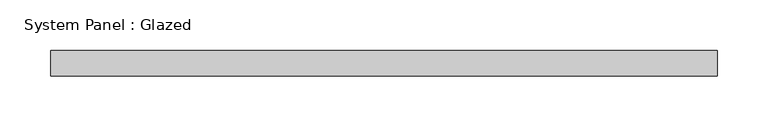
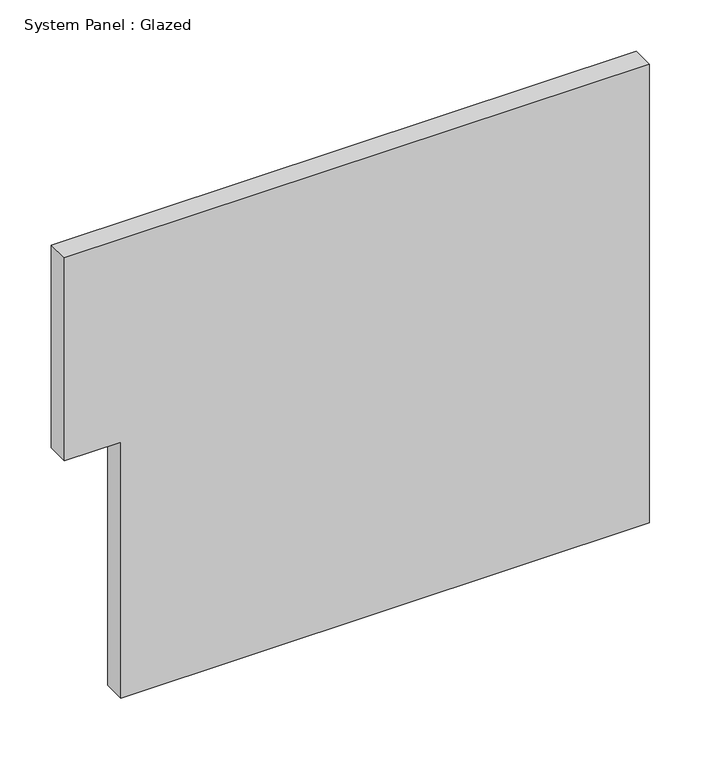
"""IFC4 building model written with IfcOpenShell, lengths in millimetres: plate geometry, System Panel : Glazed."""

import ifcopenshell
import ifcopenshell.guid

model = None  # the IFC model being written
_history = None  # IfcOwnerHistory: only IFC2X3 demands one
_inside = {}  # id of a spatial element -> (the spatial element, [elements in it])
_under = {}  # id of a project, library or spatial element -> (it, [spatial elements below it])
_declared = {}  # id of a project -> (the project, [libraries it declares])
_typed = {}  # id of a type object -> (the type object, [elements of that type])
_made_of = {}  # id of a material, layer set ... -> (it, [elements and type objects made of it])


def new_model(schema):
    """Start an empty IFC model of exactly this schema.

    Asked for "IFC4X3", IfcOpenShell would pick the latest addendum, in which some entities
    have other attributes; the version numbers below select the first issue.
    IFC2X3 requires an IfcOwnerHistory on every rooted entity: one is made here for all.
    """
    global model, _history
    if schema == "IFC4X3":
        model = ifcopenshell.file(schema_version=(4, 3, 0, 0))
    else:
        model = ifcopenshell.file(schema=schema)
    _inside.clear()
    _under.clear()
    _declared.clear()
    _typed.clear()
    _made_of.clear()
    _history = None
    if model.schema == "IFC2X3":
        org = make("IfcOrganization", Name="unknown")
        user = make(
            "IfcPersonAndOrganization",
            ThePerson=make("IfcPerson", FamilyName="unknown"),
            TheOrganization=org,
        )
        app = make(
            "IfcApplication",
            ApplicationDeveloper=org,
            Version="unknown",
            ApplicationFullName="unknown",
            ApplicationIdentifier="unknown",
        )
        _history = make(
            "IfcOwnerHistory",
            OwningUser=user,
            OwningApplication=app,
            ChangeAction="ADDED",
            CreationDate=0,
        )
    return model


def make(cls, **values):
    """One entity of the class cls with the attributes given. An attribute that is None is left unset."""
    return model.create_entity(
        cls, **{name: value for name, value in values.items() if value is not None}
    )


def rooted(cls, **values):
    """An entity with a GlobalId (a new one), such as an element, a storey or a relation."""
    return make(cls, GlobalId=ifcopenshell.guid.new(), OwnerHistory=_history, **values)


def si_unit(unit_type, name, prefix=None):
    """IfcSIUnit, for example si_unit("LENGTHUNIT", "METRE", prefix="MILLI")."""
    return make("IfcSIUnit", UnitType=unit_type, Prefix=prefix, Name=name)


def assignment(units):
    """IfcUnitAssignment: the units of a project."""
    return None if units is None else make("IfcUnitAssignment", Units=units)


def point(xyz):
    """IfcCartesianPoint."""
    return None if xyz is None else make("IfcCartesianPoint", Coordinates=xyz)


def direction(xyz):
    """IfcDirection."""
    return None if xyz is None else make("IfcDirection", DirectionRatios=xyz)


def frame(location, z_axis=None, x_axis=None):
    """IfcAxis2Placement3D, a coordinate frame: its origin and axes. An axis left out is left unset."""
    return make(
        "IfcAxis2Placement3D",
        Location=point(location),
        Axis=direction(z_axis),
        RefDirection=direction(x_axis),
    )


def origin():
    """The frame at (0, 0, 0) with its axes left unset."""
    return frame((0.0, 0.0, 0.0))


def place(relative_to, where):
    """IfcLocalPlacement: puts the frame where relative to a parent placement (None: the world)."""
    return make(
        "IfcLocalPlacement", PlacementRelTo=relative_to, RelativePlacement=where
    )


def context(
    kind, dimensions, precision=None, world=None, true_north=None, identifier=None
):
    """IfcGeometricRepresentationContext, for example the 3D "Model" context."""
    return make(
        "IfcGeometricRepresentationContext",
        ContextIdentifier=identifier,
        ContextType=kind,
        CoordinateSpaceDimension=dimensions,
        Precision=precision,
        WorldCoordinateSystem=world,
        TrueNorth=true_north,
    )


def project(units=None, contexts=None):
    """IfcProject with its units and contexts."""
    return rooted(
        "IfcProject",
        Name="project",
        RepresentationContexts=contexts,
        UnitsInContext=assignment(units),
    )


def spatial(cls, under=None, at=None, **own):
    """A site, building, storey or space (cls), placed at a placement, below another one or the project."""
    s = rooted(cls, ObjectPlacement=at, **own)
    if under is not None:
        _under.setdefault(under.id(), (under, []))[1].append(s)
    return s


def polyline(points):
    """IfcPolyline through the points."""
    return make("IfcPolyline", Points=[point(p) for p in points])


def outline(outer, holes=None, kind="AREA"):
    """IfcArbitraryClosedProfileDef: a profile drawn as a closed curve; with holes, ...WithVoids."""
    if holes is None:
        return make("IfcArbitraryClosedProfileDef", ProfileType=kind, OuterCurve=outer)
    return make(
        "IfcArbitraryProfileDefWithVoids",
        ProfileType=kind,
        OuterCurve=outer,
        InnerCurves=holes,
    )


def extrude(swept, where, along, depth):
    """IfcExtrudedAreaSolid: the profile swept, set in the frame where, extruded along a direction by depth."""
    return make(
        "IfcExtrudedAreaSolid",
        SweptArea=swept,
        Position=where,
        ExtrudedDirection=direction(along),
        Depth=depth,
    )


def shape(context_of_items, identifier, shape_type, items):
    """IfcShapeRepresentation: the items that make up one representation, for example the "Body"."""
    return make(
        "IfcShapeRepresentation",
        ContextOfItems=context_of_items,
        RepresentationIdentifier=identifier,
        RepresentationType=shape_type,
        Items=items,
    )


def source(mapping_origin, context_of_items, identifier, shape_type, items):
    """IfcRepresentationMap: a shape defined once, which mapped items show again and again."""
    return make(
        "IfcRepresentationMap",
        MappingOrigin=mapping_origin,
        MappedRepresentation=shape(context_of_items, identifier, shape_type, items),
    )


def transform(
    local_origin,
    x_axis=None,
    y_axis=None,
    z_axis=None,
    scale=None,
    scale2=None,
    scale3=None,
    uniform=True,
):
    """IfcCartesianTransformationOperator3D, or its non-uniform kind. x_axis, y_axis, z_axis: its Axis1, 2, 3."""
    if uniform:
        return make(
            "IfcCartesianTransformationOperator3D",
            Axis1=direction(x_axis),
            Axis2=direction(y_axis),
            LocalOrigin=point(local_origin),
            Scale=scale,
            Axis3=direction(z_axis),
        )
    return make(
        "IfcCartesianTransformationOperator3DnonUniform",
        Axis1=direction(x_axis),
        Axis2=direction(y_axis),
        LocalOrigin=point(local_origin),
        Scale=scale,
        Axis3=direction(z_axis),
        Scale2=scale2,
        Scale3=scale3,
    )


def mapped(mapping_source, mapping_target):
    """IfcMappedItem: shows the shape of a source again, moved by a transform."""
    return make(
        "IfcMappedItem", MappingSource=mapping_source, MappingTarget=mapping_target
    )


def made_of(thing, what):
    """Note that an element or type object is made of a material, layer set ...; save() writes the relation."""
    if what is not None:
        _made_of.setdefault(what.id(), (what, []))[1].append(thing)
    return thing


def element(
    cls,
    number,
    at=None,
    inside=None,
    cuts=None,
    type_object=None,
    material=None,
    context=None,
    identifier="Body",
    shape_type=None,
    held_by="IfcProductDefinitionShape",
    body=None,
    shapes=None,
    **own,
):
    """One element of the class cls, such as IfcWall. Its Tag is "e" and its number.

    at: its placement. inside: the storey or other place that contains it. cuts: it is an
    opening in that element (IfcRelVoidsElement). A single representation is given by context,
    identifier, shape_type and body (its items); several are given by shapes. held_by: the class
    of the entity that holds the representations. save() writes the other relations.
    """
    e = rooted(cls, Tag="e%d" % number, ObjectPlacement=at, **own)
    if body is not None:
        shapes = [shape(context, identifier, shape_type, body)]
    if shapes is not None:
        e.Representation = make(held_by, Representations=shapes)
    if inside is not None:
        _inside.setdefault(inside.id(), (inside, []))[1].append(e)
    if cuts is not None:
        rooted(
            "IfcRelVoidsElement", RelatingBuildingElement=cuts, RelatedOpeningElement=e
        )
    if type_object is not None:
        _typed.setdefault(type_object.id(), (type_object, []))[1].append(e)
    return made_of(e, material)


def aggregate(whole, parts):
    """IfcRelAggregates: a whole, such as a stair, and the parts it consists of."""
    return rooted("IfcRelAggregates", RelatingObject=whole, RelatedObjects=parts)


def save(model, path):
    """Write the relations noted so far, then the file.

    IfcRelAggregates (storeys below a building ...), IfcRelContainedInSpatialStructure (elements
    in a storey), IfcRelDefinesByType, IfcRelAssociatesMaterial and IfcRelDeclares: one each for
    every whole, place, type object, material and project.
    """
    for whole, parts in _under.values():
        aggregate(whole, parts)
    for where, things in _inside.values():
        rooted(
            "IfcRelContainedInSpatialStructure",
            RelatedElements=things,
            RelatingStructure=where,
        )
    for kind, things in _typed.values():
        rooted("IfcRelDefinesByType", RelatedObjects=things, RelatingType=kind)
    for what, things in _made_of.values():
        rooted("IfcRelAssociatesMaterial", RelatedObjects=things, RelatingMaterial=what)
    for by, libraries in _declared.values():
        rooted("IfcRelDeclares", RelatingContext=by, RelatedDefinitions=libraries)
    model.write(path)


def system_panel_glazed_78103c7b(model_context):
    return source(origin(), model_context, "Body", "SweptSolid", [
        extrude(outline(polyline([(0.0, -265.95), (0.0, 329.45), (304.8, 329.45), (546.1, 329.45), (546.1, -329.45), (304.8, -329.45), (304.8, -265.95), (0.0, -265.95)])), frame((0.0, -44.45, 0.0), z_axis=(0.0, 1.0, 0.0), x_axis=(0.0, 0.0, 1.0)), (0.0, 0.0, 1.0), 25.4),
    ])


if __name__ == "__main__":
    model = new_model("IFC4")
    model_context = context("Model", 3, world=origin())
    ifc_project = project(units=[si_unit("LENGTHUNIT", "METRE", prefix="MILLI")], contexts=[model_context])
    site = spatial("IfcSite", under=ifc_project)
    building = spatial("IfcBuilding", under=site)
    placement = place(None, origin())
    system_panel_glazed_shape = system_panel_glazed_78103c7b(model_context)
    element("IfcPlate", 1, ObjectType="System Panel : Glazed", at=placement, inside=building, context=model_context, shape_type="MappedRepresentation", body=[
        mapped(system_panel_glazed_shape, transform((0.0, 0.0, 0.0), x_axis=(1.0, 0.0, 0.0), y_axis=(0.0, 1.0, 0.0), z_axis=(0.0, 0.0, 1.0))),
    ])
    save(model, "model.ifc")

# Revit data of these elements
# Element 1 (IfcPlate, "System Panel : Glazed")
#   Materials on its faces: "Glass"
# Materials
#   "Glass": class "Glass", colour RGB 0 128 192, transparency 0.75
